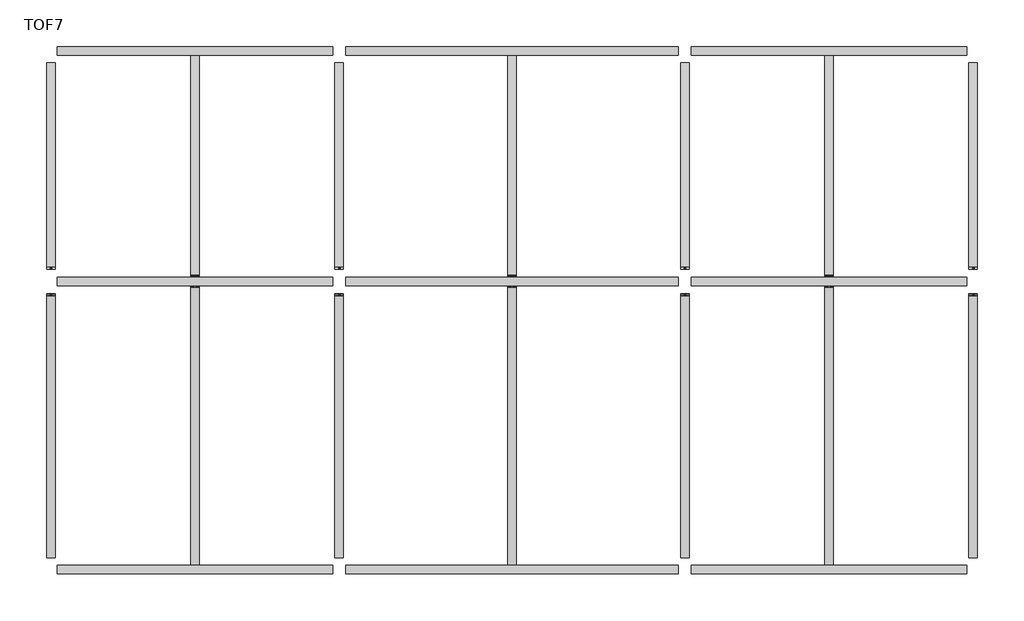
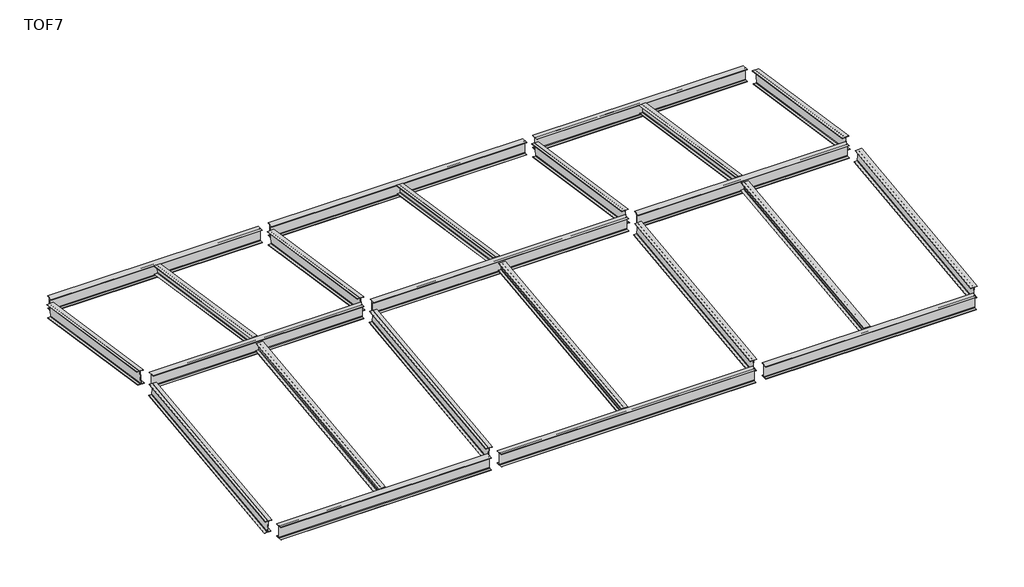
# One storey: 23 beams.
"""IFC4 building model written with IfcOpenShell, lengths in millimetres."""

import ifcopenshell
import ifcopenshell.guid

model = None  # the IFC model being written
_history = None  # IfcOwnerHistory: only IFC2X3 demands one
_inside = {}  # id of a spatial element -> (the spatial element, [elements in it])
_under = {}  # id of a project, library or spatial element -> (it, [spatial elements below it])
_declared = {}  # id of a project -> (the project, [libraries it declares])
_typed = {}  # id of a type object -> (the type object, [elements of that type])
_made_of = {}  # id of a material, layer set ... -> (it, [elements and type objects made of it])


def new_model(schema):
    """Start an empty IFC model of exactly this schema.

    Asked for "IFC4X3", IfcOpenShell would pick the latest addendum, in which some entities
    have other attributes; the version numbers below select the first issue.
    IFC2X3 requires an IfcOwnerHistory on every rooted entity: one is made here for all.
    """
    global model, _history
    if schema == "IFC4X3":
        model = ifcopenshell.file(schema_version=(4, 3, 0, 0))
    else:
        model = ifcopenshell.file(schema=schema)
    _inside.clear()
    _under.clear()
    _declared.clear()
    _typed.clear()
    _made_of.clear()
    _history = None
    if model.schema == "IFC2X3":
        org = make("IfcOrganization", Name="unknown")
        user = make(
            "IfcPersonAndOrganization",
            ThePerson=make("IfcPerson", FamilyName="unknown"),
            TheOrganization=org,
        )
        app = make(
            "IfcApplication",
            ApplicationDeveloper=org,
            Version="unknown",
            ApplicationFullName="unknown",
            ApplicationIdentifier="unknown",
        )
        _history = make(
            "IfcOwnerHistory",
            OwningUser=user,
            OwningApplication=app,
            ChangeAction="ADDED",
            CreationDate=0,
        )
    return model


def make(cls, **values):
    """One entity of the class cls with the attributes given. An attribute that is None is left unset."""
    return model.create_entity(
        cls, **{name: value for name, value in values.items() if value is not None}
    )


def rooted(cls, **values):
    """An entity with a GlobalId (a new one), such as an element, a storey or a relation."""
    return make(cls, GlobalId=ifcopenshell.guid.new(), OwnerHistory=_history, **values)


def si_unit(unit_type, name, prefix=None):
    """IfcSIUnit, for example si_unit("LENGTHUNIT", "METRE", prefix="MILLI")."""
    return make("IfcSIUnit", UnitType=unit_type, Prefix=prefix, Name=name)


def assignment(units):
    """IfcUnitAssignment: the units of a project."""
    return None if units is None else make("IfcUnitAssignment", Units=units)


def point(xyz):
    """IfcCartesianPoint."""
    return None if xyz is None else make("IfcCartesianPoint", Coordinates=xyz)


def direction(xyz):
    """IfcDirection."""
    return None if xyz is None else make("IfcDirection", DirectionRatios=xyz)


def frame(location, z_axis=None, x_axis=None):
    """IfcAxis2Placement3D, a coordinate frame: its origin and axes. An axis left out is left unset."""
    return make(
        "IfcAxis2Placement3D",
        Location=point(location),
        Axis=direction(z_axis),
        RefDirection=direction(x_axis),
    )


def frame_2d(location, x_axis=None):
    """IfcAxis2Placement2D, a coordinate frame in the plane: its origin and x axis."""
    return make(
        "IfcAxis2Placement2D", Location=point(location), RefDirection=direction(x_axis)
    )


def origin():
    """The frame at (0, 0, 0) with its axes left unset."""
    return frame((0.0, 0.0, 0.0))


def place(relative_to, where):
    """IfcLocalPlacement: puts the frame where relative to a parent placement (None: the world)."""
    return make(
        "IfcLocalPlacement", PlacementRelTo=relative_to, RelativePlacement=where
    )


def context(
    kind, dimensions, precision=None, world=None, true_north=None, identifier=None
):
    """IfcGeometricRepresentationContext, for example the 3D "Model" context."""
    return make(
        "IfcGeometricRepresentationContext",
        ContextIdentifier=identifier,
        ContextType=kind,
        CoordinateSpaceDimension=dimensions,
        Precision=precision,
        WorldCoordinateSystem=world,
        TrueNorth=true_north,
    )


def project(units=None, contexts=None):
    """IfcProject with its units and contexts."""
    return rooted(
        "IfcProject",
        Name="project",
        RepresentationContexts=contexts,
        UnitsInContext=assignment(units),
    )


def spatial(cls, under=None, at=None, **own):
    """A site, building, storey or space (cls), placed at a placement, below another one or the project."""
    s = rooted(cls, ObjectPlacement=at, **own)
    if under is not None:
        _under.setdefault(under.id(), (under, []))[1].append(s)
    return s


def polyline(points):
    """IfcPolyline through the points."""
    return make("IfcPolyline", Points=[point(p) for p in points])


def circle_curve(where, radius):
    """IfcCircle in the frame where."""
    return make("IfcCircle", Position=where, Radius=radius)


def trimmed(basis, trim1, trim2, sense, master):
    """IfcTrimmedCurve: the piece of a basis curve between two trims."""
    return make(
        "IfcTrimmedCurve",
        BasisCurve=basis,
        Trim1=trim1,
        Trim2=trim2,
        SenseAgreement=sense,
        MasterRepresentation=master,
    )


def segment(curve, same_sense, transition):
    """IfcCompositeCurveSegment."""
    return make(
        "IfcCompositeCurveSegment",
        Transition=transition,
        SameSense=same_sense,
        ParentCurve=curve,
    )


def composite_curve(segments, self_intersect=None):
    """IfcCompositeCurve: segments joined end to end."""
    return make("IfcCompositeCurve", Segments=segments, SelfIntersect=self_intersect)


def outline(outer, holes=None, kind="AREA"):
    """IfcArbitraryClosedProfileDef: a profile drawn as a closed curve; with holes, ...WithVoids."""
    if holes is None:
        return make("IfcArbitraryClosedProfileDef", ProfileType=kind, OuterCurve=outer)
    return make(
        "IfcArbitraryProfileDefWithVoids",
        ProfileType=kind,
        OuterCurve=outer,
        InnerCurves=holes,
    )


def extrude(swept, where, along, depth):
    """IfcExtrudedAreaSolid: the profile swept, set in the frame where, extruded along a direction by depth."""
    return make(
        "IfcExtrudedAreaSolid",
        SweptArea=swept,
        Position=where,
        ExtrudedDirection=direction(along),
        Depth=depth,
    )


def shape(context_of_items, identifier, shape_type, items):
    """IfcShapeRepresentation: the items that make up one representation, for example the "Body"."""
    return make(
        "IfcShapeRepresentation",
        ContextOfItems=context_of_items,
        RepresentationIdentifier=identifier,
        RepresentationType=shape_type,
        Items=items,
    )


def source(mapping_origin, context_of_items, identifier, shape_type, items):
    """IfcRepresentationMap: a shape defined once, which mapped items show again and again."""
    return make(
        "IfcRepresentationMap",
        MappingOrigin=mapping_origin,
        MappedRepresentation=shape(context_of_items, identifier, shape_type, items),
    )


def transform(
    local_origin,
    x_axis=None,
    y_axis=None,
    z_axis=None,
    scale=None,
    scale2=None,
    scale3=None,
    uniform=True,
):
    """IfcCartesianTransformationOperator3D, or its non-uniform kind. x_axis, y_axis, z_axis: its Axis1, 2, 3."""
    if uniform:
        return make(
            "IfcCartesianTransformationOperator3D",
            Axis1=direction(x_axis),
            Axis2=direction(y_axis),
            LocalOrigin=point(local_origin),
            Scale=scale,
            Axis3=direction(z_axis),
        )
    return make(
        "IfcCartesianTransformationOperator3DnonUniform",
        Axis1=direction(x_axis),
        Axis2=direction(y_axis),
        LocalOrigin=point(local_origin),
        Scale=scale,
        Axis3=direction(z_axis),
        Scale2=scale2,
        Scale3=scale3,
    )


def mapped(mapping_source, mapping_target):
    """IfcMappedItem: shows the shape of a source again, moved by a transform."""
    return make(
        "IfcMappedItem", MappingSource=mapping_source, MappingTarget=mapping_target
    )


def made_of(thing, what):
    """Note that an element or type object is made of a material, layer set ...; save() writes the relation."""
    if what is not None:
        _made_of.setdefault(what.id(), (what, []))[1].append(thing)
    return thing


def element(
    cls,
    number,
    at=None,
    inside=None,
    cuts=None,
    type_object=None,
    material=None,
    context=None,
    identifier="Body",
    shape_type=None,
    held_by="IfcProductDefinitionShape",
    body=None,
    shapes=None,
    **own,
):
    """One element of the class cls, such as IfcWall. Its Tag is "e" and its number.

    at: its placement. inside: the storey or other place that contains it. cuts: it is an
    opening in that element (IfcRelVoidsElement). A single representation is given by context,
    identifier, shape_type and body (its items); several are given by shapes. held_by: the class
    of the entity that holds the representations. save() writes the other relations.
    """
    e = rooted(cls, Tag="e%d" % number, ObjectPlacement=at, **own)
    if body is not None:
        shapes = [shape(context, identifier, shape_type, body)]
    if shapes is not None:
        e.Representation = make(held_by, Representations=shapes)
    if inside is not None:
        _inside.setdefault(inside.id(), (inside, []))[1].append(e)
    if cuts is not None:
        rooted(
            "IfcRelVoidsElement", RelatingBuildingElement=cuts, RelatedOpeningElement=e
        )
    if type_object is not None:
        _typed.setdefault(type_object.id(), (type_object, []))[1].append(e)
    return made_of(e, material)


def aggregate(whole, parts):
    """IfcRelAggregates: a whole, such as a stair, and the parts it consists of."""
    return rooted("IfcRelAggregates", RelatingObject=whole, RelatedObjects=parts)


def save(model, path):
    """Write the relations noted so far, then the file.

    IfcRelAggregates (storeys below a building ...), IfcRelContainedInSpatialStructure (elements
    in a storey), IfcRelDefinesByType, IfcRelAssociatesMaterial and IfcRelDeclares: one each for
    every whole, place, type object, material and project.
    """
    for whole, parts in _under.values():
        aggregate(whole, parts)
    for where, things in _inside.values():
        rooted(
            "IfcRelContainedInSpatialStructure",
            RelatedElements=things,
            RelatingStructure=where,
        )
    for kind, things in _typed.values():
        rooted("IfcRelDefinesByType", RelatedObjects=things, RelatingType=kind)
    for what, things in _made_of.values():
        rooted("IfcRelAssociatesMaterial", RelatedObjects=things, RelatingMaterial=what)
    for by, libraries in _declared.values():
        rooted("IfcRelDeclares", RelatingContext=by, RelatedDefinitions=libraries)
    model.write(path)


def beam_a4a24592(model_context):
    return source(origin(), model_context, "Body", "SweptSolid", [
        extrude(outline(composite_curve([segment(polyline([(75.0, -141.0), (75.0, -150.0), (-75.0, -150.0), (-75.0, -141.0), (-16.25, -141.0)]), True, "CONTINUOUS"), segment(trimmed(circle_curve(frame_2d((-16.25, -128.0)), 13.0), [point((-16.25, -141.0))], [point((-3.25, -128.0))], True, "CARTESIAN"), True, "CONTINUOUS"), segment(polyline([(-3.25, -128.0), (-3.25, 128.0)]), True, "CONTINUOUS"), segment(trimmed(circle_curve(frame_2d((-16.25, 128.0)), 13.0), [point((-3.25, 128.0))], [point((-16.25, 141.0))], True, "CARTESIAN"), True, "CONTINUOUS"), segment(polyline([(-16.25, 141.0), (-75.0, 141.0), (-75.0, 150.0), (75.0, 150.0), (75.0, 141.0), (16.25, 141.0)]), True, "CONTINUOUS"), segment(trimmed(circle_curve(frame_2d((16.25, 128.0)), 13.0), [point((16.25, 141.0))], [point((3.25, 128.0))], True, "CARTESIAN"), True, "CONTINUOUS"), segment(polyline([(3.25, 128.0), (3.25, -128.0)]), True, "CONTINUOUS"), segment(trimmed(circle_curve(frame_2d((16.25, -128.0)), 13.0), [point((3.25, -128.0))], [point((16.25, -141.0))], True, "CARTESIAN"), True, "CONTINUOUS"), segment(polyline([(16.25, -141.0), (75.0, -141.0)]), True, "CONTINUOUS")], self_intersect=False)), frame((-2387.3, 0.0, 0.0), z_axis=(1.0, 0.0, 0.0), x_axis=(0.0, 1.0, 0.0)), (0.0, 0.0, 1.0), 4774.6),
    ])


def beam_98be4253(model_context):
    return source(origin(), model_context, "Body", "SweptSolid", [
        extrude(outline(composite_curve([segment(polyline([(75.0, -141.0), (75.0, -150.0), (-75.0, -150.0), (-75.0, -141.0), (-16.25, -141.0)]), True, "CONTINUOUS"), segment(trimmed(circle_curve(frame_2d((-16.25, -128.0)), 13.0), [point((-16.25, -141.0))], [point((-3.25, -128.0))], True, "CARTESIAN"), True, "CONTINUOUS"), segment(polyline([(-3.25, -128.0), (-3.25, 128.0)]), True, "CONTINUOUS"), segment(trimmed(circle_curve(frame_2d((-16.25, 128.0)), 13.0), [point((-3.25, 128.0))], [point((-16.25, 141.0))], True, "CARTESIAN"), True, "CONTINUOUS"), segment(polyline([(-16.25, 141.0), (-75.0, 141.0), (-75.0, 150.0), (75.0, 150.0), (75.0, 141.0), (16.25, 141.0)]), True, "CONTINUOUS"), segment(trimmed(circle_curve(frame_2d((16.25, 128.0)), 13.0), [point((16.25, 141.0))], [point((3.25, 128.0))], True, "CARTESIAN"), True, "CONTINUOUS"), segment(polyline([(3.25, 128.0), (3.25, -128.0)]), True, "CONTINUOUS"), segment(trimmed(circle_curve(frame_2d((16.25, -128.0)), 13.0), [point((3.25, -128.0))], [point((16.25, -141.0))], True, "CARTESIAN"), True, "CONTINUOUS"), segment(polyline([(16.25, -141.0), (75.0, -141.0)]), True, "CONTINUOUS")], self_intersect=False)), frame((-2887.3, 0.0, 0.0), z_axis=(1.0, 0.0, 0.0), x_axis=(0.0, 1.0, 0.0)), (0.0, 0.0, 1.0), 5774.6),
    ])


def beam_c94bab30(model_context):
    return source(origin(), model_context, "Body", "SweptSolid", [
        extrude(outline(composite_curve([segment(polyline([(75.0, -141.0), (75.0, -150.0), (-75.0, -150.0), (-75.0, -141.0), (-16.25, -141.0)]), True, "CONTINUOUS"), segment(trimmed(circle_curve(frame_2d((-16.25, -128.0)), 13.0), [point((-16.25, -141.0))], [point((-3.25, -128.0))], True, "CARTESIAN"), True, "CONTINUOUS"), segment(polyline([(-3.25, -128.0), (-3.25, 128.0)]), True, "CONTINUOUS"), segment(trimmed(circle_curve(frame_2d((-16.25, 128.0)), 13.0), [point((-3.25, 128.0))], [point((-16.25, 141.0))], True, "CARTESIAN"), True, "CONTINUOUS"), segment(polyline([(-16.25, 141.0), (-75.0, 141.0), (-75.0, 150.0), (75.0, 150.0), (75.0, 141.0), (16.25, 141.0)]), True, "CONTINUOUS"), segment(trimmed(circle_curve(frame_2d((16.25, 128.0)), 13.0), [point((16.25, 141.0))], [point((3.25, 128.0))], True, "CARTESIAN"), True, "CONTINUOUS"), segment(polyline([(3.25, 128.0), (3.25, -128.0)]), True, "CONTINUOUS"), segment(trimmed(circle_curve(frame_2d((16.25, -128.0)), 13.0), [point((3.25, -128.0))], [point((16.25, -141.0))], True, "CARTESIAN"), True, "CONTINUOUS"), segment(polyline([(16.25, -141.0), (75.0, -141.0)]), True, "CONTINUOUS")], self_intersect=False)), frame((-2306.6602947, 0.0, 0.0), z_axis=(1.0, 0.0, 0.0), x_axis=(0.0, 1.0, 0.0)), (0.0, 0.0, 1.0), 4574.4611041),
    ])


def beam_d6c2ad6f(model_context):
    return source(origin(), model_context, "Body", "SweptSolid", [
        extrude(outline(composite_curve([segment(polyline([(75.0, -141.0), (75.0, -150.0), (-75.0, -150.0), (-75.0, -141.0), (-16.25, -141.0)]), True, "CONTINUOUS"), segment(trimmed(circle_curve(frame_2d((-16.25, -128.0)), 13.0), [point((-16.25, -141.0))], [point((-3.25, -128.0))], True, "CARTESIAN"), True, "CONTINUOUS"), segment(polyline([(-3.25, -128.0), (-3.25, 128.0)]), True, "CONTINUOUS"), segment(trimmed(circle_curve(frame_2d((-16.25, 128.0)), 13.0), [point((-3.25, 128.0))], [point((-16.25, 141.0))], True, "CARTESIAN"), True, "CONTINUOUS"), segment(polyline([(-16.25, 141.0), (-75.0, 141.0), (-75.0, 150.0), (75.0, 150.0), (75.0, 141.0), (16.25, 141.0)]), True, "CONTINUOUS"), segment(trimmed(circle_curve(frame_2d((16.25, 128.0)), 13.0), [point((16.25, 141.0))], [point((3.25, 128.0))], True, "CARTESIAN"), True, "CONTINUOUS"), segment(polyline([(3.25, 128.0), (3.25, -128.0)]), True, "CONTINUOUS"), segment(trimmed(circle_curve(frame_2d((16.25, -128.0)), 13.0), [point((3.25, -128.0))], [point((16.25, -141.0))], True, "CARTESIAN"), True, "CONTINUOUS"), segment(polyline([(16.25, -141.0), (75.0, -141.0)]), True, "CONTINUOUS")], self_intersect=False)), frame((-1762.4373575, 0.0, 0.0), z_axis=(1.0, 0.0, 0.0), x_axis=(0.0, 1.0, 0.0)), (0.0, 0.0, 1.0), 3574.3249285),
    ])


def beam_42108b3c(model_context):
    return source(origin(), model_context, "Body", "SweptSolid", [
        extrude(outline(composite_curve([segment(polyline([(75.0, -88.0), (75.0, -97.0), (-75.0, -97.0), (-75.0, -88.0), (-16.0, -88.0)]), True, "CONTINUOUS"), segment(trimmed(circle_curve(frame_2d((-16.0, -75.0)), 13.0), [point((-16.0, -88.0))], [point((-3.0, -75.0))], True, "CARTESIAN"), True, "CONTINUOUS"), segment(polyline([(-3.0, -75.0), (-3.0, 75.0)]), True, "CONTINUOUS"), segment(trimmed(circle_curve(frame_2d((-16.0, 75.0)), 13.0), [point((-3.0, 75.0))], [point((-16.0, 88.0))], True, "CARTESIAN"), True, "CONTINUOUS"), segment(polyline([(-16.0, 88.0), (-75.0, 88.0), (-75.0, 97.0), (75.0, 97.0), (75.0, 88.0), (16.0, 88.0)]), True, "CONTINUOUS"), segment(trimmed(circle_curve(frame_2d((16.0, 75.0)), 13.0), [point((16.0, 88.0))], [point((3.0, 75.0))], True, "CARTESIAN"), True, "CONTINUOUS"), segment(polyline([(3.0, 75.0), (3.0, -75.0)]), True, "CONTINUOUS"), segment(trimmed(circle_curve(frame_2d((16.0, -75.0)), 13.0), [point((3.0, -75.0))], [point((16.0, -88.0))], True, "CARTESIAN"), True, "CONTINUOUS"), segment(polyline([(16.0, -88.0), (75.0, -88.0)]), True, "CONTINUOUS")], self_intersect=False)), frame((-2430.7698995, 0.0, 0.0), z_axis=(1.0, 0.0, 0.0), x_axis=(0.0, 1.0, 0.0)), (0.0, 0.0, 1.0), 4837.187492),
    ])


def beam_ff5aae68(model_context):
    return source(origin(), model_context, "Body", "SweptSolid", [
        extrude(outline(composite_curve([segment(polyline([(75.0, -88.0), (75.0, -97.0), (-75.0, -97.0), (-75.0, -88.0), (-16.0, -88.0)]), True, "CONTINUOUS"), segment(trimmed(circle_curve(frame_2d((-16.0, -75.0)), 13.0), [point((-16.0, -88.0))], [point((-3.0, -75.0))], True, "CARTESIAN"), True, "CONTINUOUS"), segment(polyline([(-3.0, -75.0), (-3.0, 75.0)]), True, "CONTINUOUS"), segment(trimmed(circle_curve(frame_2d((-16.0, 75.0)), 13.0), [point((-3.0, 75.0))], [point((-16.0, 88.0))], True, "CARTESIAN"), True, "CONTINUOUS"), segment(polyline([(-16.0, 88.0), (-75.0, 88.0), (-75.0, 97.0), (75.0, 97.0), (75.0, 88.0), (16.0, 88.0)]), True, "CONTINUOUS"), segment(trimmed(circle_curve(frame_2d((16.0, 75.0)), 13.0), [point((16.0, 88.0))], [point((3.0, 75.0))], True, "CARTESIAN"), True, "CONTINUOUS"), segment(polyline([(3.0, 75.0), (3.0, -75.0)]), True, "CONTINUOUS"), segment(trimmed(circle_curve(frame_2d((16.0, -75.0)), 13.0), [point((3.0, -75.0))], [point((16.0, -88.0))], True, "CARTESIAN"), True, "CONTINUOUS"), segment(polyline([(16.0, -88.0), (75.0, -88.0)]), True, "CONTINUOUS")], self_intersect=False)), frame((-1904.7357851, 0.0, 0.0), z_axis=(1.0, 0.0, 0.0), x_axis=(0.0, 1.0, 0.0)), (0.0, 0.0, 1.0), 3840.2404002),
    ])


model = new_model("IFC4")

# Units and contexts
model_context = context("Model", 3, world=origin())
ifc_project = project(units=[si_unit("LENGTHUNIT", "METRE", prefix="MILLI")], contexts=[model_context])

# Site, building, storey
site = spatial("IfcSite", under=ifc_project)
building = spatial("IfcBuilding", under=site)
storey = spatial("IfcBuildingStorey", under=building, Name="TOF7", Elevation=12500.0)

# Beams
placement = place(None, origin())
beam_shape = beam_a4a24592(model_context)
element("IfcBeam", 1, ObjectType="0912_Steel Framing_H-KSD3502 : H_SB_AR_S02_H-300x150x6.5x9_Stair", at=placement, inside=storey, context=model_context, shape_type="MappedRepresentation", body=[
    mapped(beam_shape, transform((2500.0, 0.0, 12350.0), x_axis=(1.0, 0.0, 0.0), y_axis=(0.0, 1.0, 0.0), z_axis=(0.0, 0.0, 1.0))),
])
element("IfcBeam", 2, ObjectType="0912_Steel Framing_H-KSD3502 : H_SB_AR_S02_H-300x150x6.5x9_Stair", at=placement, inside=storey, context=model_context, shape_type="MappedRepresentation", body=[
    mapped(beam_shape, transform((13500.0, 0.0, 12350.0), x_axis=(1.0, 0.0, 0.0), y_axis=(0.0, 1.0, 0.0), z_axis=(0.0, 0.0, 1.0))),
])
element("IfcBeam", 3, ObjectType="0912_Steel Framing_H-KSD3502 : H_SB_AR_S02_H-300x150x6.5x9_Stair", at=placement, inside=storey, context=model_context, shape_type="MappedRepresentation", body=[
    mapped(beam_shape, transform((2500.0, 5000.0, 12950.0), x_axis=(1.0, 0.0, 0.0), y_axis=(0.0, 1.0, 0.0), z_axis=(0.0, 0.0, 1.0))),
])
element("IfcBeam", 4, ObjectType="0912_Steel Framing_H-KSD3502 : H_SB_AR_S02_H-300x150x6.5x9_Stair", at=placement, inside=storey, context=model_context, shape_type="MappedRepresentation", body=[
    mapped(beam_shape, transform((13500.0, 5000.0, 12950.0), x_axis=(1.0, 0.0, 0.0), y_axis=(0.0, 1.0, 0.0), z_axis=(0.0, 0.0, 1.0))),
])
element("IfcBeam", 5, ObjectType="0912_Steel Framing_H-KSD3502 : H_SB_AR_S02_H-300x150x6.5x9_Stair", at=placement, inside=storey, context=model_context, shape_type="MappedRepresentation", body=[
    mapped(beam_shape, transform((2500.0, 9000.0, 12350.0), x_axis=(1.0, 0.0, 0.0), y_axis=(0.0, 1.0, 0.0), z_axis=(0.0, 0.0, 1.0))),
])
element("IfcBeam", 6, ObjectType="0912_Steel Framing_H-KSD3502 : H_SB_AR_S02_H-300x150x6.5x9_Stair", at=placement, inside=storey, context=model_context, shape_type="MappedRepresentation", body=[
    mapped(beam_shape, transform((13500.0, 9000.0, 12350.0), x_axis=(1.0, 0.0, 0.0), y_axis=(0.0, 1.0, 0.0), z_axis=(0.0, 0.0, 1.0))),
])
beam_2_shape = beam_98be4253(model_context)
element("IfcBeam", 7, ObjectType="0912_Steel Framing_H-KSD3502 : H_SB_AR_S02_H-300x150x6.5x9_Stair", at=placement, inside=storey, context=model_context, shape_type="MappedRepresentation", body=[
    mapped(beam_2_shape, transform((8000.0, 0.0, 12350.0), x_axis=(1.0, 0.0, 0.0), y_axis=(0.0, 1.0, 0.0), z_axis=(0.0, 0.0, 1.0))),
])
element("IfcBeam", 8, ObjectType="0912_Steel Framing_H-KSD3502 : H_SB_AR_S02_H-300x150x6.5x9_Stair", at=placement, inside=storey, context=model_context, shape_type="MappedRepresentation", body=[
    mapped(beam_2_shape, transform((8000.0, 5000.0, 12950.0), x_axis=(1.0, 0.0, 0.0), y_axis=(0.0, 1.0, 0.0), z_axis=(0.0, 0.0, 1.0))),
])
element("IfcBeam", 9, ObjectType="0912_Steel Framing_H-KSD3502 : H_SB_AR_S02_H-300x150x6.5x9_Stair", at=placement, inside=storey, context=model_context, shape_type="MappedRepresentation", body=[
    mapped(beam_2_shape, transform((8000.0, 9000.0, 12350.0), x_axis=(1.0, 0.0, 0.0), y_axis=(0.0, 1.0, 0.0), z_axis=(0.0, 0.0, 1.0))),
])
beam_3_shape = beam_c94bab30(model_context)
element("IfcBeam", 10, ObjectType="0912_Steel Framing_H-KSD3502 : H_SB_AR_S02_H-300x150x6.5x9_Stair", at=placement, inside=storey, context=model_context, shape_type="MappedRepresentation", body=[
    mapped(beam_3_shape, transform((0.0, 2517.8717831, 12651.0684742), x_axis=(0.0, 0.992876838486922, 0.11914522061843107), y_axis=(-1.0, 0.0, 0.0), z_axis=(0.0, -0.11914522061843107, 0.992876838486922))),
])
element("IfcBeam", 11, ObjectType="0912_Steel Framing_H-KSD3502 : H_SB_AR_S02_H-300x150x6.5x9_Stair", at=placement, inside=storey, context=model_context, shape_type="MappedRepresentation", body=[
    mapped(beam_3_shape, transform((5000.0, 2517.8717831, 12651.0684742), x_axis=(0.0, 0.992876838486922, 0.11914522061843107), y_axis=(-1.0, 0.0, 0.0), z_axis=(0.0, -0.11914522061843107, 0.992876838486922))),
])
element("IfcBeam", 12, ObjectType="0912_Steel Framing_H-KSD3502 : H_SB_AR_S02_H-300x150x6.5x9_Stair", at=placement, inside=storey, context=model_context, shape_type="MappedRepresentation", body=[
    mapped(beam_3_shape, transform((11000.0, 2517.8717831, 12651.0684742), x_axis=(0.0, 0.992876838486922, 0.11914522061843107), y_axis=(-1.0, 0.0, 0.0), z_axis=(0.0, -0.11914522061843107, 0.992876838486922))),
])
element("IfcBeam", 13, ObjectType="0912_Steel Framing_H-KSD3502 : H_SB_AR_S02_H-300x150x6.5x9_Stair", at=placement, inside=storey, context=model_context, shape_type="MappedRepresentation", body=[
    mapped(beam_3_shape, transform((16000.0, 2517.8717831, 12651.0684742), x_axis=(0.0, 0.992876838486922, 0.11914522061843107), y_axis=(-1.0, 0.0, 0.0), z_axis=(0.0, -0.11914522061843107, 0.992876838486922))),
])
beam_4_shape = beam_d6c2ad6f(model_context)
element("IfcBeam", 14, ObjectType="0912_Steel Framing_H-KSD3502 : H_SB_AR_S02_H-300x150x6.5x9_Stair", at=placement, inside=storey, context=model_context, shape_type="MappedRepresentation", body=[
    mapped(beam_4_shape, transform((0.0, 6977.7489321, 12651.6595471), x_axis=(0.0, 0.9889363528682975, -0.1483404529302446), y_axis=(-1.0, 0.0, 0.0), z_axis=(0.0, 0.14834045293024462, 0.9889363528682976))),
])
element("IfcBeam", 15, ObjectType="0912_Steel Framing_H-KSD3502 : H_SB_AR_S02_H-300x150x6.5x9_Stair", at=placement, inside=storey, context=model_context, shape_type="MappedRepresentation", body=[
    mapped(beam_4_shape, transform((5000.0, 6977.7489321, 12651.6595471), x_axis=(0.0, 0.9889363528682975, -0.1483404529302446), y_axis=(-1.0, 0.0, 0.0), z_axis=(0.0, 0.14834045293024462, 0.9889363528682976))),
])
element("IfcBeam", 16, ObjectType="0912_Steel Framing_H-KSD3502 : H_SB_AR_S02_H-300x150x6.5x9_Stair", at=placement, inside=storey, context=model_context, shape_type="MappedRepresentation", body=[
    mapped(beam_4_shape, transform((11000.0, 6977.7489321, 12651.6595471), x_axis=(0.0, 0.9889363528682975, -0.1483404529302446), y_axis=(-1.0, 0.0, 0.0), z_axis=(0.0, 0.14834045293024462, 0.9889363528682976))),
])
element("IfcBeam", 17, ObjectType="0912_Steel Framing_H-KSD3502 : H_SB_AR_S02_H-300x150x6.5x9_Stair", at=placement, inside=storey, context=model_context, shape_type="MappedRepresentation", body=[
    mapped(beam_4_shape, transform((16000.0, 6977.7489321, 12651.6595471), x_axis=(0.0, 0.9889363528682975, -0.1483404529302446), y_axis=(-1.0, 0.0, 0.0), z_axis=(0.0, 0.14834045293024462, 0.9889363528682976))),
])
beam_5_shape = beam_42108b3c(model_context)
element("IfcBeam", 18, ObjectType="0912_Steel Framing_H-KSD3502 : H_SB_AR_S02_H-194x150x6x9_Platform", at=placement, inside=storey, context=model_context, shape_type="MappedRepresentation", body=[
    mapped(beam_5_shape, transform((2500.0, 2511.5570864, 12703.6909467), x_axis=(0.0, 0.992876838486922, 0.11914522061843107), y_axis=(-1.0, 0.0, 0.0), z_axis=(0.0, -0.11914522061843107, 0.992876838486922))),
])
element("IfcBeam", 19, ObjectType="0912_Steel Framing_H-KSD3502 : H_SB_AR_S02_H-194x150x6x9_Platform", at=placement, inside=storey, context=model_context, shape_type="MappedRepresentation", body=[
    mapped(beam_5_shape, transform((8000.0, 2511.5570864, 12703.6909467), x_axis=(0.0, 0.992876838486922, 0.11914522061843107), y_axis=(-1.0, 0.0, 0.0), z_axis=(0.0, -0.11914522061843107, 0.992876838486922))),
])
element("IfcBeam", 20, ObjectType="0912_Steel Framing_H-KSD3502 : H_SB_AR_S02_H-194x150x6x9_Platform", at=placement, inside=storey, context=model_context, shape_type="MappedRepresentation", body=[
    mapped(beam_5_shape, transform((13500.0, 2511.5570864, 12703.6909467), x_axis=(0.0, 0.992876838486922, 0.11914522061843107), y_axis=(-1.0, 0.0, 0.0), z_axis=(0.0, -0.11914522061843107, 0.992876838486922))),
])
beam_6_shape = beam_ff5aae68(model_context)
element("IfcBeam", 21, ObjectType="0912_Steel Framing_H-KSD3502 : H_SB_AR_S02_H-194x150x6x9_Platform", at=placement, inside=storey, context=model_context, shape_type="MappedRepresentation", body=[
    mapped(beam_6_shape, transform((2500.0, 6985.6109761, 12704.0731738), x_axis=(0.0, 0.9889363528682975, -0.1483404529302446), y_axis=(-1.0, 0.0, 0.0), z_axis=(0.0, 0.14834045293024462, 0.9889363528682976))),
])
element("IfcBeam", 22, ObjectType="0912_Steel Framing_H-KSD3502 : H_SB_AR_S02_H-194x150x6x9_Platform", at=placement, inside=storey, context=model_context, shape_type="MappedRepresentation", body=[
    mapped(beam_6_shape, transform((8000.0, 6985.6109761, 12704.0731738), x_axis=(0.0, 0.9889363528682975, -0.1483404529302446), y_axis=(-1.0, 0.0, 0.0), z_axis=(0.0, 0.14834045293024462, 0.9889363528682976))),
])
element("IfcBeam", 23, ObjectType="0912_Steel Framing_H-KSD3502 : H_SB_AR_S02_H-194x150x6x9_Platform", at=placement, inside=storey, context=model_context, shape_type="MappedRepresentation", body=[
    mapped(beam_6_shape, transform((13500.0, 6985.6109761, 12704.0731738), x_axis=(0.0, 0.9889363528682975, -0.1483404529302446), y_axis=(-1.0, 0.0, 0.0), z_axis=(0.0, 0.14834045293024462, 0.9889363528682976))),
])

save(model, "model.ifc")

# Revit data of these elements
# Type "0912_Steel Framing_H-KSD3502 : H_SB_AR_S02_H-300x150x6.5x9_Stair"
#   H_Q'ty Cal Type Tag = "SB-Q2"
#   H_WM Code_1 = "S01AA073-00001 |  | TON | Main Steel Structure Fabrication Work | Shelter/Building | Medium Steel - Standard |  |  |  |  |  |  | Material: (   ) | (90)KG/M>Weight≥(30)KG/M | S01AA073-00001 Main Steel Structure Fabrication Work Shelter/Building Medium Steel - Standard         | - Material: ( ASTM A36 )\n- (90)KG/M>Weight≥(30)KG/M"
#   H_WM Code_2 = "S03AA083-00001 |  | TON | Main Steel Structure Erection Work | Shelter/Building | Medium Steel |  |  |  |  |  |  | Material: (   ) | S03AA083-00001 Main Steel Structure Erection Work Shelter/Building Medium Steel         | - Material: ( ASTM A36 )"
#   H_WM Code_3 = "S01AA009-00001 |  | TON | Main Steel Structure Fabrication Work | Shelter/Building | Plates - Gusset, Stiffener, ETC | Material: (   ) | S01AA009-00001 Main Steel Structure Fabrication Work Shelter/Building Plates - Gusset, Stiffener, ETC         |"
#   H_WM Code_4 = "S41AA051-00001 |  | M2 | Steel Structure Paint Work | Shelter/Building | for Non-Fireproofed Steel Surface |  |  |  |  |  |  | Material: (   ) | S41AA051-00001 Steel Structure Paint Work Shelter/Building for Non-Fireproofed Steel Surface         |"
#   Width = 15.0 cm
#   Web Thickness = 0.65 cm
#   Web Fillet = 1.3 cm
#   Warping Constant = 107000.0 cm⁶
#   W = 0
#   Torsional Moment of Inertia = 9.9539 cm⁴
#   Section Area = 46.78 cm²
#   Plastic Modulus weak axis = 105.0 cm³
#   Plastic Modulus strong axis = 542.0 cm³
#   Perimeter = 1.17 m²/m
#   Nominal Weight = 36.70 kgf/m
#   Moment of Inertia weak axis = 508.00 cm⁴
#   Moment of Inertia strong axis = 7210.00 cm⁴
#   Height = 30.0 cm
#   Flange Thickness = 0.9 cm
#   Elastic Modulus weak axis = 67.7 cm³
#   Elastic Modulus strong axis = 481.0 cm³
#   Centroid Vertical = 15.0 cm
#   Centroid Horizontal = 7.5 cm
#   Ix = 72100000
#   Length [instance default] = 1524 mm
#   Zx = 542000
#   b = 150 mm
#   h = 300 mm
#   r = 13 mm
#   s = 6.5 mm
#   t = 9 mm
#   A = 0.004678 m²
#   Structural Material [instance default] = Steel, 45-345
#   Assembly Code = ""
# Type "0912_Steel Framing_H-KSD3502 : H_SB_AR_S02_H-194x150x6x9_Platform"
#   H_Q'ty Cal Type Tag = "SB-Q2"
#   H_WM Code_1 = "S01AA073-00001 |  | TON | Main Steel Structure Fabrication Work | Shelter/Building | Medium Steel - Standard |  |  |  |  |  |  | Material: (   ) | (90)KG/M>Weight≥(30)KG/M | S01AA073-00001 Main Steel Structure Fabrication Work Shelter/Building Medium Steel - Standard         | - Material: ( ASTM A36 )\n- (90)KG/M>Weight≥(30)KG/M"
#   H_WM Code_2 = "S03AA083-00001 |  | TON | Main Steel Structure Erection Work | Shelter/Building | Medium Steel |  |  |  |  |  |  | Material: (   ) | S03AA083-00001 Main Steel Structure Erection Work Shelter/Building Medium Steel         | - Material: ( ASTM A36 )"
#   H_WM Code_3 = "S01AA009-00001 |  | TON | Main Steel Structure Fabrication Work | Shelter/Building | Plates - Gusset, Stiffener, ETC | Material: (   ) | S01AA009-00001 Main Steel Structure Fabrication Work Shelter/Building Plates - Gusset, Stiffener, ETC         |"
#   H_WM Code_4 = "S41AA051-00001 |  | M2 | Steel Structure Paint Work | Shelter/Building | for Non-Fireproofed Steel Surface |  |  |  |  |  |  | Material: (   ) | S41AA051-00001 Steel Structure Paint Work Shelter/Building for Non-Fireproofed Steel Surface         |"
#   Width = 15.0 cm
#   Web Thickness = 0.6 cm
#   Web Fillet = 1.3 cm
#   Warping Constant = 43316.0 cm⁶
#   W = 0
#   Torsional Moment of Inertia = 8.622 cm⁴
#   Section Area = 39.01 cm²
#   Plastic Modulus weak axis = 104.0 cm³
#   Plastic Modulus strong axis = 309.0 cm³
#   Perimeter = 0.95 m²/m
#   Nominal Weight = 30.60 kgf/m
#   Moment of Inertia weak axis = 507.00 cm⁴
#   Moment of Inertia strong axis = 2690.00 cm⁴
#   Height = 19.4 cm
#   Flange Thickness = 0.9 cm
#   Elastic Modulus weak axis = 67.6 cm³
#   Elastic Modulus strong axis = 277.0 cm³
#   Centroid Vertical = 9.7 cm
#   Centroid Horizontal = 7.5 cm
#   Ix = 26900000
#   Length [instance default] = 1524 mm
#   Zx = 309000
#   b = 150 mm
#   h = 194 mm
#   r = 13 mm
#   s = 6 mm
#   t = 9 mm
#   A = 0.003901 m²
#   Structural Material [instance default] = Steel, 45-345
#   Assembly Code = ""
# Elements 1, 2, 3, 4, 5, 6, 7, 8, 9, 10, 11, 12, 13, 14, 15, 16, 17 (IfcBeam, "0912_Steel Framing_H-KSD3502 : H_SB_AR_S02_H-300x150x6.5x9_Stair")
#   Comments = ""
#   HSD_member_analysis = ""
#   Structural Material = Steel, 45-345
#   Phase Created = New Construction
#   Materials on its faces: "Steel, 45-345"
# Elements 18, 19, 20, 21, 22, 23 (IfcBeam, "0912_Steel Framing_H-KSD3502 : H_SB_AR_S02_H-194x150x6x9_Platform")
#   Comments = ""
#   HSD_member_analysis = ""
#   Structural Material = Steel, 45-345
#   Phase Created = New Construction
#   Materials on its faces: "Steel, 45-345"
# Materials
#   "Steel, 45-345": class "Metal", colour RGB 189 187 185, transparency 0, Description = "Steel 345 MPa", Cost = 0
